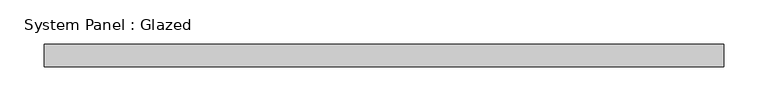
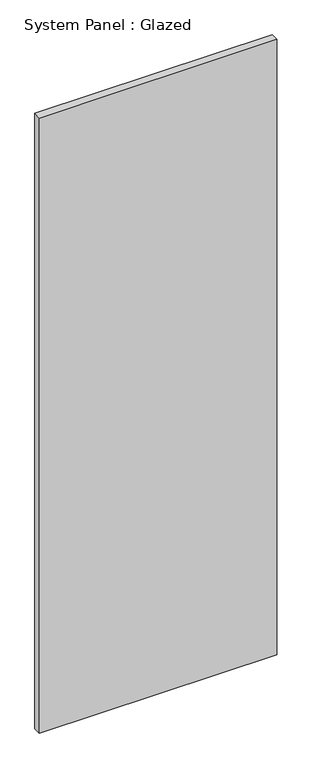
"""IFC4 building model written with IfcOpenShell, lengths in millimetres: plate geometry, System Panel : Glazed."""

from ifc_helpers import new_model, si_unit, origin, origin_with_axes, place, context, project, spatial, polyline, outline, extrude, source, transform, mapped, element, save


def system_panel_glazed_8e231006(model_context):
    return source(origin(), model_context, "Body", "SweptSolid", [
        extrude(outline(polyline([(382.3136177, 19.05), (-382.3136177, 19.05), (-382.3136177, 44.45), (382.3136177, 44.45), (382.3136177, 19.05)])), origin_with_axes(), (0.0, 0.0, 1.0), 2095.5),
    ])


if __name__ == "__main__":
    model = new_model("IFC4")
    model_context = context("Model", 3, world=origin())
    ifc_project = project(units=[si_unit("LENGTHUNIT", "METRE", prefix="MILLI")], contexts=[model_context])
    site = spatial("IfcSite", under=ifc_project)
    building = spatial("IfcBuilding", under=site)
    placement = place(None, origin())
    system_panel_glazed_shape = system_panel_glazed_8e231006(model_context)
    element("IfcPlate", 1, ObjectType="System Panel : Glazed", at=placement, inside=building, context=model_context, shape_type="MappedRepresentation", body=[
        mapped(system_panel_glazed_shape, transform((0.0, 0.0, 0.0), x_axis=(1.0, 0.0, 0.0), y_axis=(0.0, 1.0, 0.0), z_axis=(0.0, 0.0, 1.0))),
    ])
    save(model, "model.ifc")

# Revit data of these elements
# Type "System Panel : Glazed"
#   Construction Type Id = "GSP4R"
#   Analytic Construction = "1/8 in Pilkington single glazing"
#   Visual Light Transmittance = 0.9
#   Solar Heat Gain Coefficient = 0.86
#   Heat Transfer Coefficient (U) = 1.18115 BTU/(h·ft²·°F)
#   Define Thermal Properties by = 1
# Element 1 (IfcPlate, "System Panel : Glazed")
#   Materials on its faces: "Glass"
# Materials
#   "Glass": class "Glass", colour RGB 0 128 192, transparency 0.75, Description = "Soda Lime Glass", Cost = 0
